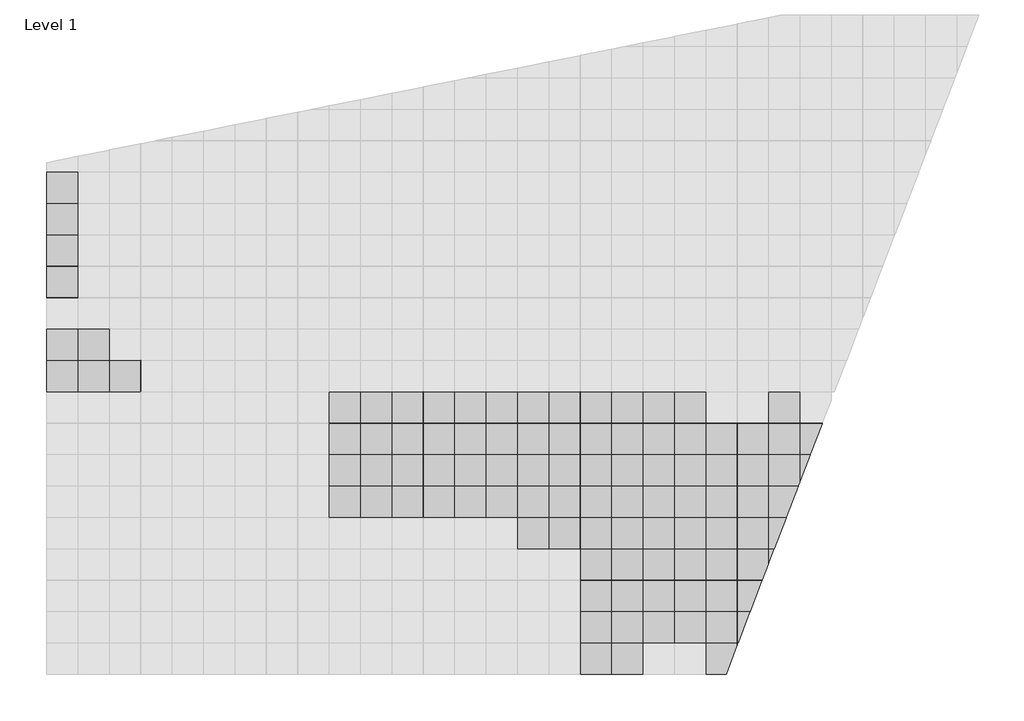
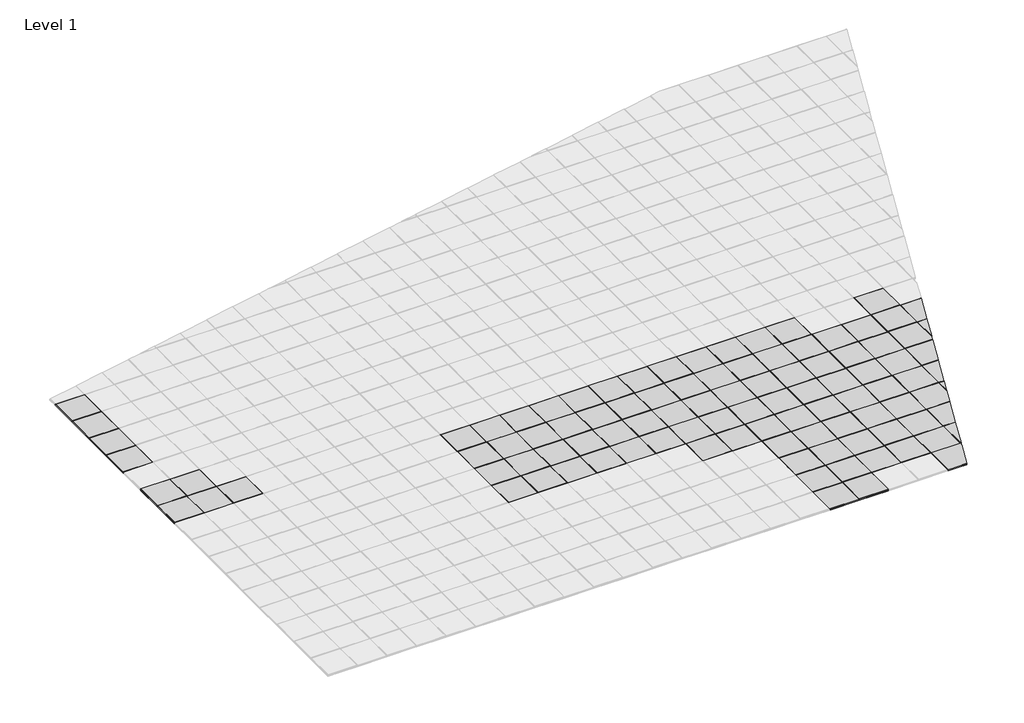
# One storey, part 4 of 18: 100 plates.
"""IFC4 building model written with IfcOpenShell, lengths in millimetres."""

import ifcopenshell
import ifcopenshell.guid

model = None  # the IFC model being written
_history = None  # IfcOwnerHistory: only IFC2X3 demands one
_inside = {}  # id of a spatial element -> (the spatial element, [elements in it])
_under = {}  # id of a project, library or spatial element -> (it, [spatial elements below it])
_declared = {}  # id of a project -> (the project, [libraries it declares])
_typed = {}  # id of a type object -> (the type object, [elements of that type])
_made_of = {}  # id of a material, layer set ... -> (it, [elements and type objects made of it])


def new_model(schema):
    """Start an empty IFC model of exactly this schema.

    Asked for "IFC4X3", IfcOpenShell would pick the latest addendum, in which some entities
    have other attributes; the version numbers below select the first issue.
    IFC2X3 requires an IfcOwnerHistory on every rooted entity: one is made here for all.
    """
    global model, _history
    if schema == "IFC4X3":
        model = ifcopenshell.file(schema_version=(4, 3, 0, 0))
    else:
        model = ifcopenshell.file(schema=schema)
    _inside.clear()
    _under.clear()
    _declared.clear()
    _typed.clear()
    _made_of.clear()
    _history = None
    if model.schema == "IFC2X3":
        org = make("IfcOrganization", Name="unknown")
        user = make(
            "IfcPersonAndOrganization",
            ThePerson=make("IfcPerson", FamilyName="unknown"),
            TheOrganization=org,
        )
        app = make(
            "IfcApplication",
            ApplicationDeveloper=org,
            Version="unknown",
            ApplicationFullName="unknown",
            ApplicationIdentifier="unknown",
        )
        _history = make(
            "IfcOwnerHistory",
            OwningUser=user,
            OwningApplication=app,
            ChangeAction="ADDED",
            CreationDate=0,
        )
    return model


def make(cls, **values):
    """One entity of the class cls with the attributes given. An attribute that is None is left unset."""
    return model.create_entity(
        cls, **{name: value for name, value in values.items() if value is not None}
    )


def rooted(cls, **values):
    """An entity with a GlobalId (a new one), such as an element, a storey or a relation."""
    return make(cls, GlobalId=ifcopenshell.guid.new(), OwnerHistory=_history, **values)


def si_unit(unit_type, name, prefix=None):
    """IfcSIUnit, for example si_unit("LENGTHUNIT", "METRE", prefix="MILLI")."""
    return make("IfcSIUnit", UnitType=unit_type, Prefix=prefix, Name=name)


def assignment(units):
    """IfcUnitAssignment: the units of a project."""
    return None if units is None else make("IfcUnitAssignment", Units=units)


def point(xyz):
    """IfcCartesianPoint."""
    return None if xyz is None else make("IfcCartesianPoint", Coordinates=xyz)


def direction(xyz):
    """IfcDirection."""
    return None if xyz is None else make("IfcDirection", DirectionRatios=xyz)


def frame(location, z_axis=None, x_axis=None):
    """IfcAxis2Placement3D, a coordinate frame: its origin and axes. An axis left out is left unset."""
    return make(
        "IfcAxis2Placement3D",
        Location=point(location),
        Axis=direction(z_axis),
        RefDirection=direction(x_axis),
    )


def origin():
    """The frame at (0, 0, 0) with its axes left unset."""
    return frame((0.0, 0.0, 0.0))


def origin_with_axes():
    """The frame at (0, 0, 0) with the z axis (0, 0, 1) and the x axis (1, 0, 0) written out."""
    return frame((0.0, 0.0, 0.0), z_axis=(0.0, 0.0, 1.0), x_axis=(1.0, 0.0, 0.0))


def place(relative_to, where):
    """IfcLocalPlacement: puts the frame where relative to a parent placement (None: the world)."""
    return make(
        "IfcLocalPlacement", PlacementRelTo=relative_to, RelativePlacement=where
    )


def context(
    kind, dimensions, precision=None, world=None, true_north=None, identifier=None
):
    """IfcGeometricRepresentationContext, for example the 3D "Model" context."""
    return make(
        "IfcGeometricRepresentationContext",
        ContextIdentifier=identifier,
        ContextType=kind,
        CoordinateSpaceDimension=dimensions,
        Precision=precision,
        WorldCoordinateSystem=world,
        TrueNorth=true_north,
    )


def project(units=None, contexts=None):
    """IfcProject with its units and contexts."""
    return rooted(
        "IfcProject",
        Name="project",
        RepresentationContexts=contexts,
        UnitsInContext=assignment(units),
    )


def spatial(cls, under=None, at=None, **own):
    """A site, building, storey or space (cls), placed at a placement, below another one or the project."""
    s = rooted(cls, ObjectPlacement=at, **own)
    if under is not None:
        _under.setdefault(under.id(), (under, []))[1].append(s)
    return s


def polyline(points):
    """IfcPolyline through the points."""
    return make("IfcPolyline", Points=[point(p) for p in points])


def outline(outer, holes=None, kind="AREA"):
    """IfcArbitraryClosedProfileDef: a profile drawn as a closed curve; with holes, ...WithVoids."""
    if holes is None:
        return make("IfcArbitraryClosedProfileDef", ProfileType=kind, OuterCurve=outer)
    return make(
        "IfcArbitraryProfileDefWithVoids",
        ProfileType=kind,
        OuterCurve=outer,
        InnerCurves=holes,
    )


def extrude(swept, where, along, depth):
    """IfcExtrudedAreaSolid: the profile swept, set in the frame where, extruded along a direction by depth."""
    return make(
        "IfcExtrudedAreaSolid",
        SweptArea=swept,
        Position=where,
        ExtrudedDirection=direction(along),
        Depth=depth,
    )


def shape(context_of_items, identifier, shape_type, items):
    """IfcShapeRepresentation: the items that make up one representation, for example the "Body"."""
    return make(
        "IfcShapeRepresentation",
        ContextOfItems=context_of_items,
        RepresentationIdentifier=identifier,
        RepresentationType=shape_type,
        Items=items,
    )


def source(mapping_origin, context_of_items, identifier, shape_type, items):
    """IfcRepresentationMap: a shape defined once, which mapped items show again and again."""
    return make(
        "IfcRepresentationMap",
        MappingOrigin=mapping_origin,
        MappedRepresentation=shape(context_of_items, identifier, shape_type, items),
    )


def transform(
    local_origin,
    x_axis=None,
    y_axis=None,
    z_axis=None,
    scale=None,
    scale2=None,
    scale3=None,
    uniform=True,
):
    """IfcCartesianTransformationOperator3D, or its non-uniform kind. x_axis, y_axis, z_axis: its Axis1, 2, 3."""
    if uniform:
        return make(
            "IfcCartesianTransformationOperator3D",
            Axis1=direction(x_axis),
            Axis2=direction(y_axis),
            LocalOrigin=point(local_origin),
            Scale=scale,
            Axis3=direction(z_axis),
        )
    return make(
        "IfcCartesianTransformationOperator3DnonUniform",
        Axis1=direction(x_axis),
        Axis2=direction(y_axis),
        LocalOrigin=point(local_origin),
        Scale=scale,
        Axis3=direction(z_axis),
        Scale2=scale2,
        Scale3=scale3,
    )


def mapped(mapping_source, mapping_target):
    """IfcMappedItem: shows the shape of a source again, moved by a transform."""
    return make(
        "IfcMappedItem", MappingSource=mapping_source, MappingTarget=mapping_target
    )


def made_of(thing, what):
    """Note that an element or type object is made of a material, layer set ...; save() writes the relation."""
    if what is not None:
        _made_of.setdefault(what.id(), (what, []))[1].append(thing)
    return thing


def element(
    cls,
    number,
    at=None,
    inside=None,
    cuts=None,
    type_object=None,
    material=None,
    context=None,
    identifier="Body",
    shape_type=None,
    held_by="IfcProductDefinitionShape",
    body=None,
    shapes=None,
    **own,
):
    """One element of the class cls, such as IfcWall. Its Tag is "e" and its number.

    at: its placement. inside: the storey or other place that contains it. cuts: it is an
    opening in that element (IfcRelVoidsElement). A single representation is given by context,
    identifier, shape_type and body (its items); several are given by shapes. held_by: the class
    of the entity that holds the representations. save() writes the other relations.
    """
    e = rooted(cls, Tag="e%d" % number, ObjectPlacement=at, **own)
    if body is not None:
        shapes = [shape(context, identifier, shape_type, body)]
    if shapes is not None:
        e.Representation = make(held_by, Representations=shapes)
    if inside is not None:
        _inside.setdefault(inside.id(), (inside, []))[1].append(e)
    if cuts is not None:
        rooted(
            "IfcRelVoidsElement", RelatingBuildingElement=cuts, RelatedOpeningElement=e
        )
    if type_object is not None:
        _typed.setdefault(type_object.id(), (type_object, []))[1].append(e)
    return made_of(e, material)


def aggregate(whole, parts):
    """IfcRelAggregates: a whole, such as a stair, and the parts it consists of."""
    return rooted("IfcRelAggregates", RelatingObject=whole, RelatedObjects=parts)


def save(model, path):
    """Write the relations noted so far, then the file.

    IfcRelAggregates (storeys below a building ...), IfcRelContainedInSpatialStructure (elements
    in a storey), IfcRelDefinesByType, IfcRelAssociatesMaterial and IfcRelDeclares: one each for
    every whole, place, type object, material and project.
    """
    for whole, parts in _under.values():
        aggregate(whole, parts)
    for where, things in _inside.values():
        rooted(
            "IfcRelContainedInSpatialStructure",
            RelatedElements=things,
            RelatingStructure=where,
        )
    for kind, things in _typed.values():
        rooted("IfcRelDefinesByType", RelatedObjects=things, RelatingType=kind)
    for what, things in _made_of.values():
        rooted("IfcRelAssociatesMaterial", RelatedObjects=things, RelatingMaterial=what)
    for by, libraries in _declared.values():
        rooted("IfcRelDeclares", RelatingContext=by, RelatedDefinitions=libraries)
    model.write(path)


def type_1_8eb2385c(model_context):
    return source(origin(), model_context, "Body", "SweptSolid", [
        extrude(outline(polyline([(1000.0, 500.0), (500.0, 500.0), (500.0, 1000.0), (1000.0, 1000.0), (1000.0, 500.0)]), holes=[polyline([(995.0, 995.0), (505.0, 995.0), (505.0, 505.0), (995.0, 505.0), (995.0, 995.0)])]), origin_with_axes(), (0.0, 0.0, 1.0), 18.0),
        extrude(outline(polyline([(505.0, 995.0), (995.0, 995.0), (995.0, 505.0), (505.0, 505.0), (505.0, 995.0)])), origin_with_axes(), (0.0, 0.0, 1.0), 20.0),
    ])


model = new_model("IFC4")

# Units and contexts
model_context = context("Model", 3, world=origin())
ifc_project = project(units=[si_unit("LENGTHUNIT", "METRE", prefix="MILLI")], contexts=[model_context])

# Site, building, storey
site = spatial("IfcSite", under=ifc_project)
building = spatial("IfcBuilding", under=site)
storey = spatial("IfcBuildingStorey", under=building, Name="Level 1", Elevation=0.0)

# Plates
placement = place(None, origin())
element("IfcPlate", 1, ObjectType="00_CPA_tegel : Type 1", at=placement, inside=storey, context=model_context, shape_type="SweptSolid", body=[
    extrude(outline(polyline([(12511.2147669, 12587.7016515), (13001.2147669, 12587.7016515), (13001.2147669, 12097.7016515), (12511.2147669, 12097.7016515), (12511.2147669, 12587.7016515)])), origin_with_axes(), (0.0, 0.0, 1.0), 20.0),
    extrude(outline(polyline([(13006.2147669, 12092.7016515), (12506.2147669, 12092.7016515), (12506.2147669, 12592.7016515), (13006.2147669, 12592.7016515), (13006.2147669, 12092.7016515)]), holes=[polyline([(13001.2147669, 12587.7016515), (12511.2147669, 12587.7016515), (12511.2147669, 12097.7016515), (13001.2147669, 12097.7016515), (13001.2147669, 12587.7016515)])]), origin_with_axes(), (0.0, 0.0, 1.0), 18.0),
])
element("IfcPlate", 2, ObjectType="00_CPA_tegel : Type 1", at=placement, inside=storey, context=model_context, shape_type="SweptSolid", body=[
    extrude(outline(polyline([(13011.2147669, 12587.7016515), (13501.2147669, 12587.7016515), (13501.2147669, 12097.7016515), (13011.2147669, 12097.7016515), (13011.2147669, 12587.7016515)])), origin_with_axes(), (0.0, 0.0, 1.0), 20.0),
    extrude(outline(polyline([(13506.2147669, 12092.7016515), (13006.2147669, 12092.7016515), (13006.2147669, 12592.7016515), (13506.2147669, 12592.7016515), (13506.2147669, 12092.7016515)]), holes=[polyline([(13501.2147669, 12587.7016515), (13011.2147669, 12587.7016515), (13011.2147669, 12097.7016515), (13501.2147669, 12097.7016515), (13501.2147669, 12587.7016515)])]), origin_with_axes(), (0.0, 0.0, 1.0), 18.0),
])
element("IfcPlate", 3, ObjectType="00_CPA_tegel : Type 1", at=placement, inside=storey, context=model_context, shape_type="SweptSolid", body=[
    extrude(outline(polyline([(14511.2147669, 12097.7016515), (14511.2147669, 12587.7016515), (15001.2147669, 12587.7016515), (15001.2147669, 12548.143408), (14828.3538669, 12097.7016515), (14511.2147669, 12097.7016515)])), origin_with_axes(), (0.0, 0.0, 1.0), 20.0),
    extrude(outline(polyline([(14506.2147669, 12592.7016515), (15006.2147669, 12592.7016515), (15006.2147669, 12561.1724318), (15001.2147669, 12548.143408), (15001.2147669, 12587.7016515), (14511.2147669, 12587.7016515), (14511.2147669, 12097.7016515), (14828.3538669, 12097.7016515), (14826.4350739, 12092.7016515), (14506.2147669, 12092.7016515), (14506.2147669, 12592.7016515)])), origin_with_axes(), (0.0, 0.0, 1.0), 18.0),
])
element("IfcPlate", 4, ObjectType="00_CPA_tegel : Type 1", at=placement, inside=storey, context=model_context, shape_type="SweptSolid", body=[
    extrude(outline(polyline([(13511.2147669, 13087.7016515), (14001.2147669, 13087.7016515), (14001.2147669, 12597.7016515), (13511.2147669, 12597.7016515), (13511.2147669, 13087.7016515)])), origin_with_axes(), (0.0, 0.0, 1.0), 20.0),
    extrude(outline(polyline([(14006.2147669, 12592.7016515), (13506.2147669, 12592.7016515), (13506.2147669, 13092.7016515), (14006.2147669, 13092.7016515), (14006.2147669, 12592.7016515)]), holes=[polyline([(14001.2147669, 13087.7016515), (13511.2147669, 13087.7016515), (13511.2147669, 12597.7016515), (14001.2147669, 12597.7016515), (14001.2147669, 13087.7016515)])]), origin_with_axes(), (0.0, 0.0, 1.0), 18.0),
])
element("IfcPlate", 5, ObjectType="00_CPA_tegel : Type 1", at=placement, inside=storey, context=model_context, shape_type="SweptSolid", body=[
    extrude(outline(polyline([(14511.2147669, 12597.7016515), (14511.2147669, 13087.7016515), (15001.2147669, 13087.7016515), (15001.2147669, 12597.7016515), (14511.2147669, 12597.7016515)])), origin_with_axes(), (0.0, 0.0, 1.0), 20.0),
    extrude(outline(polyline([(15006.2147669, 12592.7016515), (14506.2147669, 12592.7016515), (14506.2147669, 13092.7016515), (15006.2147669, 13092.7016515), (15006.2147669, 12592.7016515)]), holes=[polyline([(15001.2147669, 13087.7016515), (14511.2147669, 13087.7016515), (14511.2147669, 12597.7016515), (15001.2147669, 12597.7016515), (15001.2147669, 13087.7016515)])]), origin_with_axes(), (0.0, 0.0, 1.0), 18.0),
])
element("IfcPlate", 6, ObjectType="00_CPA_tegel : Type 1", at=placement, inside=storey, context=model_context, shape_type="SweptSolid", body=[
    extrude(outline(polyline([(15011.2147669, 12597.7016515), (15011.2147669, 13087.7016515), (15208.2748857, 13087.7016515), (15020.2331693, 12597.7016515), (15011.2147669, 12597.7016515)])), origin_with_axes(), (0.0, 0.0, 1.0), 20.0),
    extrude(outline(polyline([(15006.2147669, 12592.7016515), (15006.2147669, 13092.7016515), (15210.1936787, 13092.7016515), (15208.2748857, 13087.7016515), (15011.2147669, 13087.7016515), (15011.2147669, 12597.7016515), (15020.2331693, 12597.7016515), (15018.3143763, 12592.7016515), (15006.2147669, 12592.7016515)])), origin_with_axes(), (0.0, 0.0, 1.0), 18.0),
])
element("IfcPlate", 7, ObjectType="00_CPA_tegel : Type 1", at=placement, inside=storey, context=model_context, shape_type="SweptSolid", body=[
    extrude(outline(polyline([(13511.2147669, 13587.7016515), (14001.2147669, 13587.7016515), (14001.2147669, 13097.7016515), (13511.2147669, 13097.7016515), (13511.2147669, 13587.7016515)])), origin_with_axes(), (0.0, 0.0, 1.0), 20.0),
    extrude(outline(polyline([(14006.2147669, 13092.7016515), (13506.2147669, 13092.7016515), (13506.2147669, 13592.7016515), (14006.2147669, 13592.7016515), (14006.2147669, 13092.7016515)]), holes=[polyline([(14001.2147669, 13587.7016515), (13511.2147669, 13587.7016515), (13511.2147669, 13097.7016515), (14001.2147669, 13097.7016515), (14001.2147669, 13587.7016515)])]), origin_with_axes(), (0.0, 0.0, 1.0), 18.0),
])
element("IfcPlate", 8, ObjectType="00_CPA_tegel : Type 1", at=placement, inside=storey, context=model_context, shape_type="SweptSolid", body=[
    extrude(outline(polyline([(14011.2147669, 13587.7016515), (14501.2147669, 13587.7016515), (14501.2147669, 13097.7016515), (14011.2147669, 13097.7016515), (14011.2147669, 13587.7016515)])), origin_with_axes(), (0.0, 0.0, 1.0), 20.0),
    extrude(outline(polyline([(14506.2147669, 13092.7016515), (14006.2147669, 13092.7016515), (14006.2147669, 13592.7016515), (14506.2147669, 13592.7016515), (14506.2147669, 13092.7016515)]), holes=[polyline([(14501.2147669, 13587.7016515), (14011.2147669, 13587.7016515), (14011.2147669, 13097.7016515), (14501.2147669, 13097.7016515), (14501.2147669, 13587.7016515)])]), origin_with_axes(), (0.0, 0.0, 1.0), 18.0),
])
element("IfcPlate", 9, ObjectType="00_CPA_tegel : Type 1", at=placement, inside=storey, context=model_context, shape_type="SweptSolid", body=[
    extrude(outline(polyline([(15011.2147669, 13097.7016515), (15011.2147669, 13587.7016515), (15400.1541881, 13587.7016515), (15212.1124717, 13097.7016515), (15011.2147669, 13097.7016515)])), origin_with_axes(), (0.0, 0.0, 1.0), 20.0),
    extrude(outline(polyline([(15006.2147669, 13092.7016515), (15006.2147669, 13592.7016515), (15402.0729811, 13592.7016515), (15400.1541881, 13587.7016515), (15011.2147669, 13587.7016515), (15011.2147669, 13097.7016515), (15212.1124717, 13097.7016515), (15210.1936787, 13092.7016515), (15006.2147669, 13092.7016515)])), origin_with_axes(), (0.0, 0.0, 1.0), 18.0),
])
element("IfcPlate", 10, ObjectType="00_CPA_tegel : Type 1", at=placement, inside=storey, context=model_context, shape_type="SweptSolid", body=[
    extrude(outline(polyline([(14011.2147669, 14087.7016515), (14501.2147669, 14087.7016515), (14501.2147669, 13597.7016515), (14011.2147669, 13597.7016515), (14011.2147669, 14087.7016515)])), origin_with_axes(), (0.0, 0.0, 1.0), 20.0),
    extrude(outline(polyline([(14506.2147669, 13592.7016515), (14006.2147669, 13592.7016515), (14006.2147669, 14092.7016515), (14506.2147669, 14092.7016515), (14506.2147669, 13592.7016515)]), holes=[polyline([(14501.2147669, 14087.7016515), (14011.2147669, 14087.7016515), (14011.2147669, 13597.7016515), (14501.2147669, 13597.7016515), (14501.2147669, 14087.7016515)])]), origin_with_axes(), (0.0, 0.0, 1.0), 18.0),
])
element("IfcPlate", 11, ObjectType="00_CPA_tegel : Type 1", at=placement, inside=storey, context=model_context, shape_type="SweptSolid", body=[
    extrude(outline(polyline([(15011.2147669, 13597.7016515), (15011.2147669, 14087.7016515), (15501.2147669, 14087.7016515), (15501.2147669, 13851.0457891), (15403.9917741, 13597.7016515), (15011.2147669, 13597.7016515)])), origin_with_axes(), (0.0, 0.0, 1.0), 20.0),
    extrude(outline(polyline([(15006.2147669, 14092.7016515), (15506.2147669, 14092.7016515), (15506.2147669, 13864.074813), (15501.2147669, 13851.0457891), (15501.2147669, 14087.7016515), (15011.2147669, 14087.7016515), (15011.2147669, 13597.7016515), (15403.9917741, 13597.7016515), (15402.0729811, 13592.7016515), (15006.2147669, 13592.7016515), (15006.2147669, 14092.7016515)])), origin_with_axes(), (0.0, 0.0, 1.0), 18.0),
])
element("IfcPlate", 12, ObjectType="00_CPA_tegel : Type 1", at=placement, inside=storey, context=model_context, shape_type="SweptSolid", body=[
    extrude(outline(polyline([(15511.2147669, 13877.1038368), (15511.2147669, 14087.7016515), (15592.0334905, 14087.7016515), (15511.2147669, 13877.1038368)])), origin_with_axes(), (0.0, 0.0, 1.0), 20.0),
    extrude(outline(polyline([(15506.2147669, 14092.7016515), (15593.9522835, 14092.7016515), (15592.0334905, 14087.7016515), (15511.2147669, 14087.7016515), (15511.2147669, 13877.1038368), (15506.2147669, 13864.074813), (15506.2147669, 14092.7016515)])), origin_with_axes(), (0.0, 0.0, 1.0), 18.0),
])
element("IfcPlate", 13, ObjectType="00_CPA_tegel : Type 1", at=placement, inside=storey, context=model_context, shape_type="SweptSolid", body=[
    extrude(outline(polyline([(14011.2147669, 14587.7016515), (14501.2147669, 14587.7016515), (14501.2147669, 14097.7016515), (14011.2147669, 14097.7016515), (14011.2147669, 14587.7016515)])), origin_with_axes(), (0.0, 0.0, 1.0), 20.0),
    extrude(outline(polyline([(14506.2147669, 14092.7016515), (14006.2147669, 14092.7016515), (14006.2147669, 14592.7016515), (14506.2147669, 14592.7016515), (14506.2147669, 14092.7016515)]), holes=[polyline([(14501.2147669, 14587.7016515), (14011.2147669, 14587.7016515), (14011.2147669, 14097.7016515), (14501.2147669, 14097.7016515), (14501.2147669, 14587.7016515)])]), origin_with_axes(), (0.0, 0.0, 1.0), 18.0),
])
element("IfcPlate", 14, ObjectType="00_CPA_tegel : Type 1", at=placement, inside=storey, context=model_context, shape_type="SweptSolid", body=[
    extrude(outline(polyline([(15511.2147669, 14097.7016515), (15511.2147669, 14587.7016515), (15783.9127929, 14587.7016515), (15595.8710765, 14097.7016515), (15511.2147669, 14097.7016515)])), origin_with_axes(), (0.0, 0.0, 1.0), 20.0),
    extrude(outline(polyline([(15506.2147669, 14092.7016515), (15506.2147669, 14592.7016515), (15785.8315859, 14592.7016515), (15783.9127929, 14587.7016515), (15511.2147669, 14587.7016515), (15511.2147669, 14097.7016515), (15595.8710765, 14097.7016515), (15593.9522835, 14092.7016515), (15506.2147669, 14092.7016515)])), origin_with_axes(), (0.0, 0.0, 1.0), 18.0),
])
element("IfcPlate", 15, ObjectType="00_CPA_tegel : Type 1", at=placement, inside=storey, context=model_context, shape_type="SweptSolid", body=[
    extrude(outline(polyline([(14011.2147669, 15087.7016515), (14501.2147669, 15087.7016515), (14501.2147669, 14597.7016515), (14011.2147669, 14597.7016515), (14011.2147669, 15087.7016515)])), origin_with_axes(), (0.0, 0.0, 1.0), 20.0),
    extrude(outline(polyline([(14506.2147669, 14592.7016515), (14006.2147669, 14592.7016515), (14006.2147669, 15092.7016515), (14506.2147669, 15092.7016515), (14506.2147669, 14592.7016515)]), holes=[polyline([(14501.2147669, 15087.7016515), (14011.2147669, 15087.7016515), (14011.2147669, 14597.7016515), (14501.2147669, 14597.7016515), (14501.2147669, 15087.7016515)])]), origin_with_axes(), (0.0, 0.0, 1.0), 18.0),
])
element("IfcPlate", 16, ObjectType="00_CPA_tegel : Type 1", at=placement, inside=storey, context=model_context, shape_type="SweptSolid", body=[
    extrude(outline(polyline([(14511.2147669, 15087.7016515), (15001.2147669, 15087.7016515), (15001.2147669, 14597.7016515), (14511.2147669, 14597.7016515), (14511.2147669, 15087.7016515)])), origin_with_axes(), (0.0, 0.0, 1.0), 20.0),
    extrude(outline(polyline([(15006.2147669, 14592.7016515), (14506.2147669, 14592.7016515), (14506.2147669, 15092.7016515), (15006.2147669, 15092.7016515), (15006.2147669, 14592.7016515)]), holes=[polyline([(15001.2147669, 15087.7016515), (14511.2147669, 15087.7016515), (14511.2147669, 14597.7016515), (15001.2147669, 14597.7016515), (15001.2147669, 15087.7016515)])]), origin_with_axes(), (0.0, 0.0, 1.0), 18.0),
])
element("IfcPlate", 17, ObjectType="00_CPA_tegel : Type 1", at=placement, inside=storey, context=model_context, shape_type="SweptSolid", body=[
    extrude(outline(polyline([(15511.2147669, 14597.7016515), (15511.2147669, 15087.7016515), (15975.7920953, 15087.7016515), (15787.7503789, 14597.7016515), (15511.2147669, 14597.7016515)])), origin_with_axes(), (0.0, 0.0, 1.0), 20.0),
    extrude(outline(polyline([(15506.2147669, 14592.7016515), (15506.2147669, 15092.7016515), (15977.7108883, 15092.7016515), (15975.7920953, 15087.7016515), (15511.2147669, 15087.7016515), (15511.2147669, 14597.7016515), (15787.7503789, 14597.7016515), (15785.8315859, 14592.7016515), (15506.2147669, 14592.7016515)])), origin_with_axes(), (0.0, 0.0, 1.0), 18.0),
])
element("IfcPlate", 18, ObjectType="00_CPA_tegel : Type 1", at=placement, inside=storey, context=model_context, shape_type="SweptSolid", body=[
    extrude(outline(polyline([(14511.2147669, 15587.7016515), (15001.2147669, 15587.7016515), (15001.2147669, 15097.7016515), (14511.2147669, 15097.7016515), (14511.2147669, 15587.7016515)])), origin_with_axes(), (0.0, 0.0, 1.0), 20.0),
    extrude(outline(polyline([(15006.2147669, 15092.7016515), (14506.2147669, 15092.7016515), (14506.2147669, 15592.7016515), (15006.2147669, 15592.7016515), (15006.2147669, 15092.7016515)]), holes=[polyline([(15001.2147669, 15587.7016515), (14511.2147669, 15587.7016515), (14511.2147669, 15097.7016515), (15001.2147669, 15097.7016515), (15001.2147669, 15587.7016515)])]), origin_with_axes(), (0.0, 0.0, 1.0), 18.0),
])
element("IfcPlate", 19, ObjectType="00_CPA_tegel : Type 1", at=placement, inside=storey, context=model_context, shape_type="SweptSolid", body=[
    extrude(outline(polyline([(15511.2147669, 15097.7016515), (15511.2147669, 15587.7016515), (16001.2147669, 15587.7016515), (16001.2147669, 15153.9481703), (15979.6296813, 15097.7016515), (15511.2147669, 15097.7016515)])), origin_with_axes(), (0.0, 0.0, 1.0), 20.0),
    extrude(outline(polyline([(15506.2147669, 15592.7016515), (16006.2147669, 15592.7016515), (16006.2147669, 15166.9771941), (16001.2147669, 15153.9481703), (16001.2147669, 15587.7016515), (15511.2147669, 15587.7016515), (15511.2147669, 15097.7016515), (15979.6296813, 15097.7016515), (15977.7108883, 15092.7016515), (15506.2147669, 15092.7016515), (15506.2147669, 15592.7016515)])), origin_with_axes(), (0.0, 0.0, 1.0), 18.0),
])
element("IfcPlate", 20, ObjectType="00_CPA_tegel : Type 1", at=placement, inside=storey, context=model_context, shape_type="SweptSolid", body=[
    extrude(outline(polyline([(16011.2147669, 15180.0062179), (16011.2147669, 15587.7016515), (16167.6713977, 15587.7016515), (16011.2147669, 15180.0062179)])), origin_with_axes(), (0.0, 0.0, 1.0), 20.0),
    extrude(outline(polyline([(16006.2147669, 15592.7016515), (16169.5901907, 15592.7016515), (16167.6713977, 15587.7016515), (16011.2147669, 15587.7016515), (16011.2147669, 15180.0062179), (16006.2147669, 15166.9771941), (16006.2147669, 15592.7016515)])), origin_with_axes(), (0.0, 0.0, 1.0), 18.0),
])
element("IfcPlate", 21, ObjectType="00_CPA_tegel : Type 1", at=placement, inside=storey, context=model_context, shape_type="SweptSolid", body=[
    extrude(outline(polyline([(14511.2147669, 16087.7016515), (15001.2147669, 16087.7016515), (15001.2147669, 15597.7016515), (14511.2147669, 15597.7016515), (14511.2147669, 16087.7016515)])), origin_with_axes(), (0.0, 0.0, 1.0), 20.0),
    extrude(outline(polyline([(15006.2147669, 15592.7016515), (14506.2147669, 15592.7016515), (14506.2147669, 16092.7016515), (15006.2147669, 16092.7016515), (15006.2147669, 15592.7016515)]), holes=[polyline([(15001.2147669, 16087.7016515), (14511.2147669, 16087.7016515), (14511.2147669, 15597.7016515), (15001.2147669, 15597.7016515), (15001.2147669, 16087.7016515)])]), origin_with_axes(), (0.0, 0.0, 1.0), 18.0),
])
element("IfcPlate", 22, ObjectType="00_CPA_tegel : Type 1", at=placement, inside=storey, context=model_context, shape_type="SweptSolid", body=[
    extrude(outline(polyline([(16011.2147669, 15597.7016515), (16011.2147669, 16087.7016515), (16359.5507001, 16087.7016515), (16171.5089837, 15597.7016515), (16011.2147669, 15597.7016515)])), origin_with_axes(), (0.0, 0.0, 1.0), 20.0),
    extrude(outline(polyline([(16006.2147669, 15592.7016515), (16006.2147669, 16092.7016515), (16361.4694931, 16092.7016515), (16359.5507001, 16087.7016515), (16011.2147669, 16087.7016515), (16011.2147669, 15597.7016515), (16171.5089837, 15597.7016515), (16169.5901907, 15592.7016515), (16006.2147669, 15592.7016515)])), origin_with_axes(), (0.0, 0.0, 1.0), 18.0),
])
type_1_shape = type_1_8eb2385c(model_context)
element("IfcPlate", 23, ObjectType="00_CPA_tegel : Type 1", at=placement, inside=storey, context=model_context, shape_type="MappedRepresentation", body=[
    mapped(type_1_shape, transform((8006.2147669, 14092.7016515, 0.0), x_axis=(1.0000000000000002, 0.0, 0.0), y_axis=(0.0, 1.0000000000000002, 0.0), z_axis=(0.0, 0.0, 1.0))),
])
element("IfcPlate", 24, ObjectType="00_CPA_tegel : Type 1", at=placement, inside=storey, context=model_context, shape_type="MappedRepresentation", body=[
    mapped(type_1_shape, transform((8006.2147669, 14592.7016515, 0.0), x_axis=(1.0000000000000002, 0.0, 0.0), y_axis=(0.0, 1.0000000000000002, 0.0), z_axis=(0.0, 0.0, 1.0))),
])
element("IfcPlate", 25, ObjectType="00_CPA_tegel : Type 1", at=placement, inside=storey, context=model_context, shape_type="MappedRepresentation", body=[
    mapped(type_1_shape, transform((8006.2147669, 15092.7016515, 0.0), x_axis=(1.0000000000000002, 0.0, 0.0), y_axis=(0.0, 1.0000000000000002, 0.0), z_axis=(0.0, 0.0, 1.0))),
])
element("IfcPlate", 26, ObjectType="00_CPA_tegel : Type 1", at=placement, inside=storey, context=model_context, shape_type="MappedRepresentation", body=[
    mapped(type_1_shape, transform((8006.2147669, 15592.7016515, 0.0), x_axis=(1.0000000000000002, 0.0, 0.0), y_axis=(0.0, 1.0000000000000002, 0.0), z_axis=(0.0, 0.0, 1.0))),
])
element("IfcPlate", 27, ObjectType="00_CPA_tegel : Type 1", at=placement, inside=storey, context=model_context, shape_type="MappedRepresentation", body=[
    mapped(type_1_shape, transform((8506.2147669, 14092.7016515, 0.0), x_axis=(1.0000000000000002, 0.0, 0.0), y_axis=(0.0, 1.0000000000000002, 0.0), z_axis=(0.0, 0.0, 1.0))),
])
element("IfcPlate", 28, ObjectType="00_CPA_tegel : Type 1", at=placement, inside=storey, context=model_context, shape_type="MappedRepresentation", body=[
    mapped(type_1_shape, transform((9006.2147669, 14092.7016515, 0.0), x_axis=(1.0000000000000002, 0.0, 0.0), y_axis=(0.0, 1.0000000000000002, 0.0), z_axis=(0.0, 0.0, 1.0))),
])
element("IfcPlate", 29, ObjectType="00_CPA_tegel : Type 1", at=placement, inside=storey, context=model_context, shape_type="MappedRepresentation", body=[
    mapped(type_1_shape, transform((8506.2147669, 14592.7016515, 0.0), x_axis=(1.0000000000000002, 0.0, 0.0), y_axis=(0.0, 1.0000000000000002, 0.0), z_axis=(0.0, 0.0, 1.0))),
])
element("IfcPlate", 30, ObjectType="00_CPA_tegel : Type 1", at=placement, inside=storey, context=model_context, shape_type="MappedRepresentation", body=[
    mapped(type_1_shape, transform((9006.2147669, 14592.7016515, 0.0), x_axis=(1.0000000000000002, 0.0, 0.0), y_axis=(0.0, 1.0000000000000002, 0.0), z_axis=(0.0, 0.0, 1.0))),
])
element("IfcPlate", 31, ObjectType="00_CPA_tegel : Type 1", at=placement, inside=storey, context=model_context, shape_type="MappedRepresentation", body=[
    mapped(type_1_shape, transform((8506.2147669, 15092.7016515, 0.0), x_axis=(1.0000000000000002, 0.0, 0.0), y_axis=(0.0, 1.0000000000000002, 0.0), z_axis=(0.0, 0.0, 1.0))),
])
element("IfcPlate", 32, ObjectType="00_CPA_tegel : Type 1", at=placement, inside=storey, context=model_context, shape_type="MappedRepresentation", body=[
    mapped(type_1_shape, transform((9006.2147669, 15092.7016515, 0.0), x_axis=(1.0000000000000002, 0.0, 0.0), y_axis=(0.0, 1.0000000000000002, 0.0), z_axis=(0.0, 0.0, 1.0))),
])
element("IfcPlate", 33, ObjectType="00_CPA_tegel : Type 1", at=placement, inside=storey, context=model_context, shape_type="MappedRepresentation", body=[
    mapped(type_1_shape, transform((8506.2147669, 15592.7016515, 0.0), x_axis=(1.0000000000000002, 0.0, 0.0), y_axis=(0.0, 1.0000000000000002, 0.0), z_axis=(0.0, 0.0, 1.0))),
])
element("IfcPlate", 34, ObjectType="00_CPA_tegel : Type 1", at=placement, inside=storey, context=model_context, shape_type="MappedRepresentation", body=[
    mapped(type_1_shape, transform((9006.2147669, 15592.7016515, 0.0), x_axis=(1.0000000000000002, 0.0, 0.0), y_axis=(0.0, 1.0000000000000002, 0.0), z_axis=(0.0, 0.0, 1.0))),
])
element("IfcPlate", 35, ObjectType="00_CPA_tegel : Type 1", at=placement, inside=storey, context=model_context, shape_type="MappedRepresentation", body=[
    mapped(type_1_shape, transform((9506.2147669, 15092.7016515, 0.0), x_axis=(1.0000000000000002, 0.0, 0.0), y_axis=(0.0, 1.0000000000000002, 0.0), z_axis=(0.0, 0.0, 1.0))),
])
element("IfcPlate", 36, ObjectType="00_CPA_tegel : Type 1", at=placement, inside=storey, context=model_context, shape_type="MappedRepresentation", body=[
    mapped(type_1_shape, transform((9506.2147669, 15592.7016515, 0.0), x_axis=(1.0000000000000002, 0.0, 0.0), y_axis=(0.0, 1.0000000000000002, 0.0), z_axis=(0.0, 0.0, 1.0))),
])
element("IfcPlate", 37, ObjectType="00_CPA_tegel : Type 1", at=placement, inside=storey, context=model_context, shape_type="MappedRepresentation", body=[
    mapped(type_1_shape, transform((3506.2147669, 16092.7016515, 0.0), x_axis=(1.0000000000000002, 0.0, 0.0), y_axis=(0.0, 1.0000000000000002, 0.0), z_axis=(0.0, 0.0, 1.0))),
])
element("IfcPlate", 38, ObjectType="00_CPA_tegel : Type 1", at=placement, inside=storey, context=model_context, shape_type="MappedRepresentation", body=[
    mapped(type_1_shape, transform((4006.2147669, 16092.7016515, 0.0), x_axis=(1.0000000000000002, 0.0, 0.0), y_axis=(0.0, 1.0000000000000002, 0.0), z_axis=(0.0, 0.0, 1.0))),
])
element("IfcPlate", 39, ObjectType="00_CPA_tegel : Type 1", at=placement, inside=storey, context=model_context, shape_type="MappedRepresentation", body=[
    mapped(type_1_shape, transform((4506.2147669, 16092.7016515, 0.0), x_axis=(1.0000000000000002, 0.0, 0.0), y_axis=(0.0, 1.0000000000000002, 0.0), z_axis=(0.0, 0.0, 1.0))),
])
element("IfcPlate", 40, ObjectType="00_CPA_tegel : Type 1", at=placement, inside=storey, context=model_context, shape_type="MappedRepresentation", body=[
    mapped(type_1_shape, transform((9506.2147669, 14092.7016515, 0.0), x_axis=(1.0000000000000002, 0.0, 0.0), y_axis=(0.0, 1.0000000000000002, 0.0), z_axis=(0.0, 0.0, 1.0))),
])
element("IfcPlate", 41, ObjectType="00_CPA_tegel : Type 1", at=placement, inside=storey, context=model_context, shape_type="MappedRepresentation", body=[
    mapped(type_1_shape, transform((9506.2147669, 14592.7016515, 0.0), x_axis=(1.0000000000000002, 0.0, 0.0), y_axis=(0.0, 1.0000000000000002, 0.0), z_axis=(0.0, 0.0, 1.0))),
])
element("IfcPlate", 42, ObjectType="00_CPA_tegel : Type 1", at=placement, inside=storey, context=model_context, shape_type="MappedRepresentation", body=[
    mapped(type_1_shape, transform((10006.2147669, 15592.7016515, 0.0), x_axis=(1.0000000000000002, 0.0, 0.0), y_axis=(0.0, 1.0000000000000002, 0.0), z_axis=(0.0, 0.0, 1.0))),
])
element("IfcPlate", 43, ObjectType="00_CPA_tegel : Type 1", at=placement, inside=storey, context=model_context, shape_type="MappedRepresentation", body=[
    mapped(type_1_shape, transform((10006.2147669, 14092.7016515, 0.0), x_axis=(1.0000000000000002, 0.0, 0.0), y_axis=(0.0, 1.0000000000000002, 0.0), z_axis=(0.0, 0.0, 1.0))),
])
element("IfcPlate", 44, ObjectType="00_CPA_tegel : Type 1", at=placement, inside=storey, context=model_context, shape_type="MappedRepresentation", body=[
    mapped(type_1_shape, transform((10006.2147669, 14592.7016515, 0.0), x_axis=(1.0000000000000002, 0.0, 0.0), y_axis=(0.0, 1.0000000000000002, 0.0), z_axis=(0.0, 0.0, 1.0))),
])
element("IfcPlate", 45, ObjectType="00_CPA_tegel : Type 1", at=placement, inside=storey, context=model_context, shape_type="MappedRepresentation", body=[
    mapped(type_1_shape, transform((10006.2147669, 15092.7016515, 0.0), x_axis=(1.0000000000000002, 0.0, 0.0), y_axis=(0.0, 1.0000000000000002, 0.0), z_axis=(0.0, 0.0, 1.0))),
])
element("IfcPlate", 46, ObjectType="00_CPA_tegel : Type 1", at=placement, inside=storey, context=model_context, shape_type="MappedRepresentation", body=[
    mapped(type_1_shape, transform((10506.2147669, 15092.7016515, 0.0), x_axis=(1.0000000000000002, 0.0, 0.0), y_axis=(0.0, 1.0000000000000002, 0.0), z_axis=(0.0, 0.0, 1.0))),
])
element("IfcPlate", 47, ObjectType="00_CPA_tegel : Type 1", at=placement, inside=storey, context=model_context, shape_type="MappedRepresentation", body=[
    mapped(type_1_shape, transform((10506.2147669, 15592.7016515, 0.0), x_axis=(1.0000000000000002, 0.0, 0.0), y_axis=(0.0, 1.0000000000000002, 0.0), z_axis=(0.0, 0.0, 1.0))),
])
element("IfcPlate", 48, ObjectType="00_CPA_tegel : Type 1", at=placement, inside=storey, context=model_context, shape_type="MappedRepresentation", body=[
    mapped(type_1_shape, transform((3506.2147669, 16592.7016515, 0.0), x_axis=(1.0000000000000002, 0.0, 0.0), y_axis=(0.0, 1.0000000000000002, 0.0), z_axis=(0.0, 0.0, 1.0))),
])
element("IfcPlate", 49, ObjectType="00_CPA_tegel : Type 1", at=placement, inside=storey, context=model_context, shape_type="MappedRepresentation", body=[
    mapped(type_1_shape, transform((4006.2147669, 16592.7016515, 0.0), x_axis=(1.0000000000000002, 0.0, 0.0), y_axis=(0.0, 1.0000000000000002, 0.0), z_axis=(0.0, 0.0, 1.0))),
])
element("IfcPlate", 50, ObjectType="00_CPA_tegel : Type 1", at=placement, inside=storey, context=model_context, shape_type="MappedRepresentation", body=[
    mapped(type_1_shape, transform((12006.2147669, 12092.7016515, 0.0), x_axis=(1.0000000000000002, 0.0, 0.0), y_axis=(0.0, 1.0000000000000002, 0.0), z_axis=(0.0, 0.0, 1.0))),
])
element("IfcPlate", 51, ObjectType="00_CPA_tegel : Type 1", at=placement, inside=storey, context=model_context, shape_type="MappedRepresentation", body=[
    mapped(type_1_shape, transform((12506.2147669, 12092.7016515, 0.0), x_axis=(1.0000000000000002, 0.0, 0.0), y_axis=(0.0, 1.0000000000000002, 0.0), z_axis=(0.0, 0.0, 1.0))),
])
element("IfcPlate", 52, ObjectType="00_CPA_tegel : Type 1", at=placement, inside=storey, context=model_context, shape_type="MappedRepresentation", body=[
    mapped(type_1_shape, transform((13506.2147669, 12092.7016515, 0.0), x_axis=(1.0000000000000002, 0.0, 0.0), y_axis=(0.0, 1.0000000000000002, 0.0), z_axis=(0.0, 0.0, 1.0))),
])
element("IfcPlate", 53, ObjectType="00_CPA_tegel : Type 1", at=placement, inside=storey, context=model_context, shape_type="MappedRepresentation", body=[
    mapped(type_1_shape, transform((12006.2147669, 12592.7016515, 0.0), x_axis=(1.0000000000000002, 0.0, 0.0), y_axis=(0.0, 1.0000000000000002, 0.0), z_axis=(0.0, 0.0, 1.0))),
])
element("IfcPlate", 54, ObjectType="00_CPA_tegel : Type 1", at=placement, inside=storey, context=model_context, shape_type="MappedRepresentation", body=[
    mapped(type_1_shape, transform((12506.2147669, 12592.7016515, 0.0), x_axis=(1.0000000000000002, 0.0, 0.0), y_axis=(0.0, 1.0000000000000002, 0.0), z_axis=(0.0, 0.0, 1.0))),
])
element("IfcPlate", 55, ObjectType="00_CPA_tegel : Type 1", at=placement, inside=storey, context=model_context, shape_type="MappedRepresentation", body=[
    mapped(type_1_shape, transform((14006.2147669, 12592.7016515, 0.0), x_axis=(1.0000000000000002, 0.0, 0.0), y_axis=(0.0, 1.0000000000000002, 0.0), z_axis=(0.0, 0.0, 1.0))),
])
element("IfcPlate", 56, ObjectType="00_CPA_tegel : Type 1", at=placement, inside=storey, context=model_context, shape_type="MappedRepresentation", body=[
    mapped(type_1_shape, transform((12006.2147669, 13092.7016515, 0.0), x_axis=(1.0000000000000002, 0.0, 0.0), y_axis=(0.0, 1.0000000000000002, 0.0), z_axis=(0.0, 0.0, 1.0))),
])
element("IfcPlate", 57, ObjectType="00_CPA_tegel : Type 1", at=placement, inside=storey, context=model_context, shape_type="MappedRepresentation", body=[
    mapped(type_1_shape, transform((12506.2147669, 13092.7016515, 0.0), x_axis=(1.0000000000000002, 0.0, 0.0), y_axis=(0.0, 1.0000000000000002, 0.0), z_axis=(0.0, 0.0, 1.0))),
])
element("IfcPlate", 58, ObjectType="00_CPA_tegel : Type 1", at=placement, inside=storey, context=model_context, shape_type="MappedRepresentation", body=[
    mapped(type_1_shape, transform((13006.2147669, 13092.7016515, 0.0), x_axis=(1.0000000000000002, 0.0, 0.0), y_axis=(0.0, 1.0000000000000002, 0.0), z_axis=(0.0, 0.0, 1.0))),
])
element("IfcPlate", 59, ObjectType="00_CPA_tegel : Type 1", at=placement, inside=storey, context=model_context, shape_type="MappedRepresentation", body=[
    mapped(type_1_shape, transform((14006.2147669, 13092.7016515, 0.0), x_axis=(1.0000000000000002, 0.0, 0.0), y_axis=(0.0, 1.0000000000000002, 0.0), z_axis=(0.0, 0.0, 1.0))),
])
element("IfcPlate", 60, ObjectType="00_CPA_tegel : Type 1", at=placement, inside=storey, context=model_context, shape_type="MappedRepresentation", body=[
    mapped(type_1_shape, transform((11006.2147669, 13592.7016515, 0.0), x_axis=(1.0000000000000002, 0.0, 0.0), y_axis=(0.0, 1.0000000000000002, 0.0), z_axis=(0.0, 0.0, 1.0))),
])
element("IfcPlate", 61, ObjectType="00_CPA_tegel : Type 1", at=placement, inside=storey, context=model_context, shape_type="MappedRepresentation", body=[
    mapped(type_1_shape, transform((11506.2147669, 13592.7016515, 0.0), x_axis=(1.0000000000000002, 0.0, 0.0), y_axis=(0.0, 1.0000000000000002, 0.0), z_axis=(0.0, 0.0, 1.0))),
])
element("IfcPlate", 62, ObjectType="00_CPA_tegel : Type 1", at=placement, inside=storey, context=model_context, shape_type="MappedRepresentation", body=[
    mapped(type_1_shape, transform((12006.2147669, 13592.7016515, 0.0), x_axis=(1.0000000000000002, 0.0, 0.0), y_axis=(0.0, 1.0000000000000002, 0.0), z_axis=(0.0, 0.0, 1.0))),
])
element("IfcPlate", 63, ObjectType="00_CPA_tegel : Type 1", at=placement, inside=storey, context=model_context, shape_type="MappedRepresentation", body=[
    mapped(type_1_shape, transform((12506.2147669, 13592.7016515, 0.0), x_axis=(1.0000000000000002, 0.0, 0.0), y_axis=(0.0, 1.0000000000000002, 0.0), z_axis=(0.0, 0.0, 1.0))),
])
element("IfcPlate", 64, ObjectType="00_CPA_tegel : Type 1", at=placement, inside=storey, context=model_context, shape_type="MappedRepresentation", body=[
    mapped(type_1_shape, transform((13006.2147669, 13592.7016515, 0.0), x_axis=(1.0000000000000002, 0.0, 0.0), y_axis=(0.0, 1.0000000000000002, 0.0), z_axis=(0.0, 0.0, 1.0))),
])
element("IfcPlate", 65, ObjectType="00_CPA_tegel : Type 1", at=placement, inside=storey, context=model_context, shape_type="MappedRepresentation", body=[
    mapped(type_1_shape, transform((14006.2147669, 13592.7016515, 0.0), x_axis=(1.0000000000000002, 0.0, 0.0), y_axis=(0.0, 1.0000000000000002, 0.0), z_axis=(0.0, 0.0, 1.0))),
])
element("IfcPlate", 66, ObjectType="00_CPA_tegel : Type 1", at=placement, inside=storey, context=model_context, shape_type="MappedRepresentation", body=[
    mapped(type_1_shape, transform((14506.2147669, 13592.7016515, 0.0), x_axis=(1.0000000000000002, 0.0, 0.0), y_axis=(0.0, 1.0000000000000002, 0.0), z_axis=(0.0, 0.0, 1.0))),
])
element("IfcPlate", 67, ObjectType="00_CPA_tegel : Type 1", at=placement, inside=storey, context=model_context, shape_type="MappedRepresentation", body=[
    mapped(type_1_shape, transform((10506.2147669, 14092.7016515, 0.0), x_axis=(1.0000000000000002, 0.0, 0.0), y_axis=(0.0, 1.0000000000000002, 0.0), z_axis=(0.0, 0.0, 1.0))),
])
element("IfcPlate", 68, ObjectType="00_CPA_tegel : Type 1", at=placement, inside=storey, context=model_context, shape_type="MappedRepresentation", body=[
    mapped(type_1_shape, transform((11006.2147669, 14092.7016515, 0.0), x_axis=(1.0000000000000002, 0.0, 0.0), y_axis=(0.0, 1.0000000000000002, 0.0), z_axis=(0.0, 0.0, 1.0))),
])
element("IfcPlate", 69, ObjectType="00_CPA_tegel : Type 1", at=placement, inside=storey, context=model_context, shape_type="MappedRepresentation", body=[
    mapped(type_1_shape, transform((11506.2147669, 14092.7016515, 0.0), x_axis=(1.0000000000000002, 0.0, 0.0), y_axis=(0.0, 1.0000000000000002, 0.0), z_axis=(0.0, 0.0, 1.0))),
])
element("IfcPlate", 70, ObjectType="00_CPA_tegel : Type 1", at=placement, inside=storey, context=model_context, shape_type="MappedRepresentation", body=[
    mapped(type_1_shape, transform((12006.2147669, 14092.7016515, 0.0), x_axis=(1.0000000000000002, 0.0, 0.0), y_axis=(0.0, 1.0000000000000002, 0.0), z_axis=(0.0, 0.0, 1.0))),
])
element("IfcPlate", 71, ObjectType="00_CPA_tegel : Type 1", at=placement, inside=storey, context=model_context, shape_type="MappedRepresentation", body=[
    mapped(type_1_shape, transform((12506.2147669, 14092.7016515, 0.0), x_axis=(1.0000000000000002, 0.0, 0.0), y_axis=(0.0, 1.0000000000000002, 0.0), z_axis=(0.0, 0.0, 1.0))),
])
element("IfcPlate", 72, ObjectType="00_CPA_tegel : Type 1", at=placement, inside=storey, context=model_context, shape_type="MappedRepresentation", body=[
    mapped(type_1_shape, transform((13006.2147669, 14092.7016515, 0.0), x_axis=(1.0000000000000002, 0.0, 0.0), y_axis=(0.0, 1.0000000000000002, 0.0), z_axis=(0.0, 0.0, 1.0))),
])
element("IfcPlate", 73, ObjectType="00_CPA_tegel : Type 1", at=placement, inside=storey, context=model_context, shape_type="MappedRepresentation", body=[
    mapped(type_1_shape, transform((14506.2147669, 14092.7016515, 0.0), x_axis=(1.0000000000000002, 0.0, 0.0), y_axis=(0.0, 1.0000000000000002, 0.0), z_axis=(0.0, 0.0, 1.0))),
])
element("IfcPlate", 74, ObjectType="00_CPA_tegel : Type 1", at=placement, inside=storey, context=model_context, shape_type="MappedRepresentation", body=[
    mapped(type_1_shape, transform((10506.2147669, 14592.7016515, 0.0), x_axis=(1.0000000000000002, 0.0, 0.0), y_axis=(0.0, 1.0000000000000002, 0.0), z_axis=(0.0, 0.0, 1.0))),
])
element("IfcPlate", 75, ObjectType="00_CPA_tegel : Type 1", at=placement, inside=storey, context=model_context, shape_type="MappedRepresentation", body=[
    mapped(type_1_shape, transform((11006.2147669, 14592.7016515, 0.0), x_axis=(1.0000000000000002, 0.0, 0.0), y_axis=(0.0, 1.0000000000000002, 0.0), z_axis=(0.0, 0.0, 1.0))),
])
element("IfcPlate", 76, ObjectType="00_CPA_tegel : Type 1", at=placement, inside=storey, context=model_context, shape_type="MappedRepresentation", body=[
    mapped(type_1_shape, transform((11506.2147669, 14592.7016515, 0.0), x_axis=(1.0000000000000002, 0.0, 0.0), y_axis=(0.0, 1.0000000000000002, 0.0), z_axis=(0.0, 0.0, 1.0))),
])
element("IfcPlate", 77, ObjectType="00_CPA_tegel : Type 1", at=placement, inside=storey, context=model_context, shape_type="MappedRepresentation", body=[
    mapped(type_1_shape, transform((12006.2147669, 14592.7016515, 0.0), x_axis=(1.0000000000000002, 0.0, 0.0), y_axis=(0.0, 1.0000000000000002, 0.0), z_axis=(0.0, 0.0, 1.0))),
])
element("IfcPlate", 78, ObjectType="00_CPA_tegel : Type 1", at=placement, inside=storey, context=model_context, shape_type="MappedRepresentation", body=[
    mapped(type_1_shape, transform((12506.2147669, 14592.7016515, 0.0), x_axis=(1.0000000000000002, 0.0, 0.0), y_axis=(0.0, 1.0000000000000002, 0.0), z_axis=(0.0, 0.0, 1.0))),
])
element("IfcPlate", 79, ObjectType="00_CPA_tegel : Type 1", at=placement, inside=storey, context=model_context, shape_type="MappedRepresentation", body=[
    mapped(type_1_shape, transform((13006.2147669, 14592.7016515, 0.0), x_axis=(1.0000000000000002, 0.0, 0.0), y_axis=(0.0, 1.0000000000000002, 0.0), z_axis=(0.0, 0.0, 1.0))),
])
element("IfcPlate", 80, ObjectType="00_CPA_tegel : Type 1", at=placement, inside=storey, context=model_context, shape_type="MappedRepresentation", body=[
    mapped(type_1_shape, transform((13506.2147669, 14592.7016515, 0.0), x_axis=(1.0000000000000002, 0.0, 0.0), y_axis=(0.0, 1.0000000000000002, 0.0), z_axis=(0.0, 0.0, 1.0))),
])
element("IfcPlate", 81, ObjectType="00_CPA_tegel : Type 1", at=placement, inside=storey, context=model_context, shape_type="MappedRepresentation", body=[
    mapped(type_1_shape, transform((14506.2147669, 14592.7016515, 0.0), x_axis=(1.0000000000000002, 0.0, 0.0), y_axis=(0.0, 1.0000000000000002, 0.0), z_axis=(0.0, 0.0, 1.0))),
])
element("IfcPlate", 82, ObjectType="00_CPA_tegel : Type 1", at=placement, inside=storey, context=model_context, shape_type="MappedRepresentation", body=[
    mapped(type_1_shape, transform((11006.2147669, 15092.7016515, 0.0), x_axis=(1.0000000000000002, 0.0, 0.0), y_axis=(0.0, 1.0000000000000002, 0.0), z_axis=(0.0, 0.0, 1.0))),
])
element("IfcPlate", 83, ObjectType="00_CPA_tegel : Type 1", at=placement, inside=storey, context=model_context, shape_type="MappedRepresentation", body=[
    mapped(type_1_shape, transform((11506.2147669, 15092.7016515, 0.0), x_axis=(1.0000000000000002, 0.0, 0.0), y_axis=(0.0, 1.0000000000000002, 0.0), z_axis=(0.0, 0.0, 1.0))),
])
element("IfcPlate", 84, ObjectType="00_CPA_tegel : Type 1", at=placement, inside=storey, context=model_context, shape_type="MappedRepresentation", body=[
    mapped(type_1_shape, transform((12006.2147669, 15092.7016515, 0.0), x_axis=(1.0000000000000002, 0.0, 0.0), y_axis=(0.0, 1.0000000000000002, 0.0), z_axis=(0.0, 0.0, 1.0))),
])
element("IfcPlate", 85, ObjectType="00_CPA_tegel : Type 1", at=placement, inside=storey, context=model_context, shape_type="MappedRepresentation", body=[
    mapped(type_1_shape, transform((12506.2147669, 15092.7016515, 0.0), x_axis=(1.0000000000000002, 0.0, 0.0), y_axis=(0.0, 1.0000000000000002, 0.0), z_axis=(0.0, 0.0, 1.0))),
])
element("IfcPlate", 86, ObjectType="00_CPA_tegel : Type 1", at=placement, inside=storey, context=model_context, shape_type="MappedRepresentation", body=[
    mapped(type_1_shape, transform((13006.2147669, 15092.7016515, 0.0), x_axis=(1.0000000000000002, 0.0, 0.0), y_axis=(0.0, 1.0000000000000002, 0.0), z_axis=(0.0, 0.0, 1.0))),
])
element("IfcPlate", 87, ObjectType="00_CPA_tegel : Type 1", at=placement, inside=storey, context=model_context, shape_type="MappedRepresentation", body=[
    mapped(type_1_shape, transform((13506.2147669, 15092.7016515, 0.0), x_axis=(1.0000000000000002, 0.0, 0.0), y_axis=(0.0, 1.0000000000000002, 0.0), z_axis=(0.0, 0.0, 1.0))),
])
element("IfcPlate", 88, ObjectType="00_CPA_tegel : Type 1", at=placement, inside=storey, context=model_context, shape_type="MappedRepresentation", body=[
    mapped(type_1_shape, transform((14506.2147669, 15092.7016515, 0.0), x_axis=(1.0000000000000002, 0.0, 0.0), y_axis=(0.0, 1.0000000000000002, 0.0), z_axis=(0.0, 0.0, 1.0))),
])
element("IfcPlate", 89, ObjectType="00_CPA_tegel : Type 1", at=placement, inside=storey, context=model_context, shape_type="MappedRepresentation", body=[
    mapped(type_1_shape, transform((15006.2147669, 15092.7016515, 0.0), x_axis=(1.0000000000000002, 0.0, 0.0), y_axis=(0.0, 1.0000000000000002, 0.0), z_axis=(0.0, 0.0, 1.0))),
])
element("IfcPlate", 90, ObjectType="00_CPA_tegel : Type 1", at=placement, inside=storey, context=model_context, shape_type="MappedRepresentation", body=[
    mapped(type_1_shape, transform((11006.2147669, 15592.7016515, 0.0), x_axis=(1.0000000000000002, 0.0, 0.0), y_axis=(0.0, 1.0000000000000002, 0.0), z_axis=(0.0, 0.0, 1.0))),
])
element("IfcPlate", 91, ObjectType="00_CPA_tegel : Type 1", at=placement, inside=storey, context=model_context, shape_type="MappedRepresentation", body=[
    mapped(type_1_shape, transform((11506.2147669, 15592.7016515, 0.0), x_axis=(1.0000000000000002, 0.0, 0.0), y_axis=(0.0, 1.0000000000000002, 0.0), z_axis=(0.0, 0.0, 1.0))),
])
element("IfcPlate", 92, ObjectType="00_CPA_tegel : Type 1", at=placement, inside=storey, context=model_context, shape_type="MappedRepresentation", body=[
    mapped(type_1_shape, transform((12006.2147669, 15592.7016515, 0.0), x_axis=(1.0000000000000002, 0.0, 0.0), y_axis=(0.0, 1.0000000000000002, 0.0), z_axis=(0.0, 0.0, 1.0))),
])
element("IfcPlate", 93, ObjectType="00_CPA_tegel : Type 1", at=placement, inside=storey, context=model_context, shape_type="MappedRepresentation", body=[
    mapped(type_1_shape, transform((12506.2147669, 15592.7016515, 0.0), x_axis=(1.0000000000000002, 0.0, 0.0), y_axis=(0.0, 1.0000000000000002, 0.0), z_axis=(0.0, 0.0, 1.0))),
])
element("IfcPlate", 94, ObjectType="00_CPA_tegel : Type 1", at=placement, inside=storey, context=model_context, shape_type="MappedRepresentation", body=[
    mapped(type_1_shape, transform((13006.2147669, 15592.7016515, 0.0), x_axis=(1.0000000000000002, 0.0, 0.0), y_axis=(0.0, 1.0000000000000002, 0.0), z_axis=(0.0, 0.0, 1.0))),
])
element("IfcPlate", 95, ObjectType="00_CPA_tegel : Type 1", at=placement, inside=storey, context=model_context, shape_type="MappedRepresentation", body=[
    mapped(type_1_shape, transform((13506.2147669, 15592.7016515, 0.0), x_axis=(1.0000000000000002, 0.0, 0.0), y_axis=(0.0, 1.0000000000000002, 0.0), z_axis=(0.0, 0.0, 1.0))),
])
element("IfcPlate", 96, ObjectType="00_CPA_tegel : Type 1", at=placement, inside=storey, context=model_context, shape_type="MappedRepresentation", body=[
    mapped(type_1_shape, transform((15006.2147669, 15592.7016515, 0.0), x_axis=(1.0000000000000002, 0.0, 0.0), y_axis=(0.0, 1.0000000000000002, 0.0), z_axis=(0.0, 0.0, 1.0))),
])
element("IfcPlate", 97, ObjectType="00_CPA_tegel : Type 1", at=placement, inside=storey, context=model_context, shape_type="MappedRepresentation", body=[
    mapped(type_1_shape, transform((3506.2147669, 17592.7016515, 0.0), x_axis=(1.0000000000000002, 0.0, 0.0), y_axis=(0.0, 1.0000000000000002, 0.0), z_axis=(0.0, 0.0, 1.0))),
])
element("IfcPlate", 98, ObjectType="00_CPA_tegel : Type 1", at=placement, inside=storey, context=model_context, shape_type="MappedRepresentation", body=[
    mapped(type_1_shape, transform((3506.2147669, 18092.7016515, 0.0), x_axis=(1.0000000000000002, 0.0, 0.0), y_axis=(0.0, 1.0000000000000002, 0.0), z_axis=(0.0, 0.0, 1.0))),
])
element("IfcPlate", 99, ObjectType="00_CPA_tegel : Type 1", at=placement, inside=storey, context=model_context, shape_type="MappedRepresentation", body=[
    mapped(type_1_shape, transform((3506.2147669, 18592.7016515, 0.0), x_axis=(1.0000000000000002, 0.0, 0.0), y_axis=(0.0, 1.0000000000000002, 0.0), z_axis=(0.0, 0.0, 1.0))),
])
element("IfcPlate", 100, ObjectType="00_CPA_tegel : Type 1", at=placement, inside=storey, context=model_context, shape_type="MappedRepresentation", body=[
    mapped(type_1_shape, transform((3506.2147669, 19092.7016515, 0.0), x_axis=(1.0000000000000002, 0.0, 0.0), y_axis=(0.0, 1.0000000000000002, 0.0), z_axis=(0.0, 0.0, 1.0))),
])

save(model, "model.ifc")

# Revit data of these elements
# Type "00_CPA_tegel : Type 1"
#   Voegdikte = 18 mm
#   Tegeldikte = 20 mm
#   HalveVoegbreedte = 5 mm
#   Voeg = 20_voeg
#   MateriaalSteen = 300_hardsteen_zwart
# Elements 1, 2, 4, 7, 8, 10, 13, 15, 16, 18, 21, 23, 24, 25, 26, 27, 28, 29, 30, 31, 32, 33, 34, 35, 36, 37, 38, 39, 40, 41, 42, 43, 44, 45, 46, 47, 48, 49, 50, 51, 52, 53, 54, 55, 56, 57, 58, 59, 60, 61, 62, 63, 64, 65, 66, 67, 68, 69, 70, 71, 72, 73, 74, 75, 76, 77, 78, 79, 80, 81, 82, 83, 84, 85, 86, 87, 88, 89, 90, 91, 92, 93, 94, 95, 96, 97, 98, 99, 100 (IfcPlate, "00_CPA_tegel : Type 1")
#   Area = 0.25 m²
#   Phase Created = New Construction
#   Materials on its faces: "20_voeg", "300_hardsteen_zwart"
# Element 3 (IfcPlate, "00_CPA_tegel : Type 1")
#   Area = 0.180874 m²
#   Phase Created = New Construction
#   Materials on its faces: "20_voeg", "300_hardsteen_zwart"
# Element 5 (IfcPlate, "00_CPA_tegel : Type 1")
#   Area = 0.247667 m²
#   Phase Created = New Construction
#   Materials on its faces: "20_voeg", "300_hardsteen_zwart"
# Element 6 (IfcPlate, "00_CPA_tegel : Type 1")
#   Area = 0.0291464 m²
#   Phase Created = New Construction
#   Materials on its faces: "20_voeg", "300_hardsteen_zwart"
# Element 9 (IfcPlate, "00_CPA_tegel : Type 1")
#   Area = 0.122754 m²
#   Phase Created = New Construction
#   Materials on its faces: "20_voeg", "300_hardsteen_zwart"
# Element 11 (IfcPlate, "00_CPA_tegel : Type 1")
#   Area = 0.217246 m²
#   Phase Created = New Construction
#   Materials on its faces: "20_voeg", "300_hardsteen_zwart"
# Element 12 (IfcPlate, "00_CPA_tegel : Type 1")
#   Area = 0.00144695 m²
#   Phase Created = New Construction
#   Materials on its faces: "20_voeg", "300_hardsteen_zwart"
# Element 14 (IfcPlate, "00_CPA_tegel : Type 1")
#   Area = 0.0646321 m²
#   Phase Created = New Construction
#   Materials on its faces: "20_voeg", "300_hardsteen_zwart"
# Element 17 (IfcPlate, "00_CPA_tegel : Type 1")
#   Area = 0.160572 m²
#   Phase Created = New Construction
#   Materials on its faces: "20_voeg", "300_hardsteen_zwart"
# Element 19 (IfcPlate, "00_CPA_tegel : Type 1")
#   Area = 0.241042 m²
#   Phase Created = New Construction
#   Materials on its faces: "20_voeg", "300_hardsteen_zwart"
# Element 20 (IfcPlate, "00_CPA_tegel : Type 1")
#   Area = 0.0154693 m²
#   Phase Created = New Construction
#   Materials on its faces: "20_voeg", "300_hardsteen_zwart"
# Element 22 (IfcPlate, "00_CPA_tegel : Type 1")
#   Area = 0.102451 m²
#   Phase Created = New Construction
#   Materials on its faces: "20_voeg", "300_hardsteen_zwart"
# Materials
#   "20_voeg": class "Concrete", colour RGB 86 86 86, transparency 0, Manufacturer = "RevitGG", URL = "www.revitgg.nl", Description = "zandcement, generiek materiaal", Cost = 0
#   "300_hardsteen_zwart": class "Generic", colour RGB 15 15 15, transparency 0, Description = "kalkzandsteen", Cost = 0
